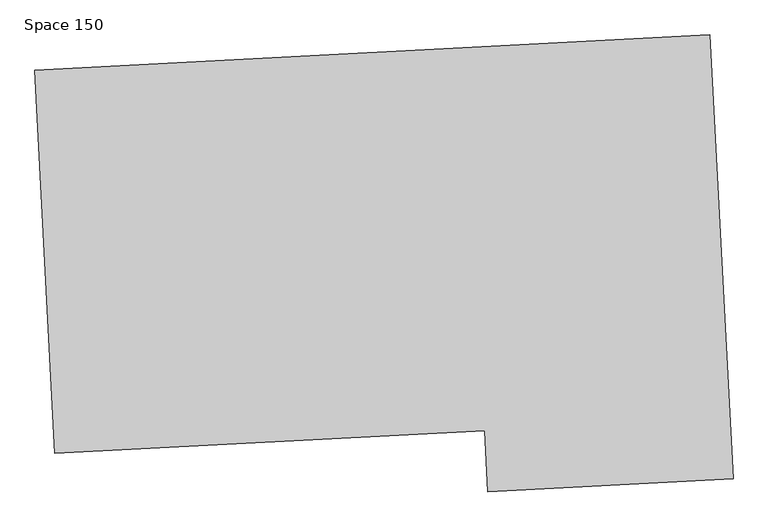
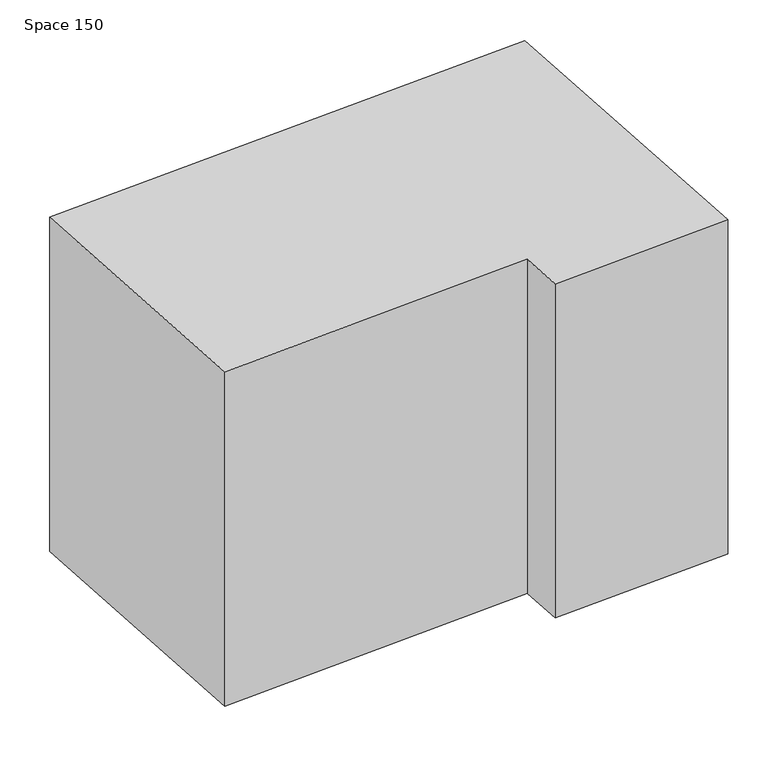
"""IFC4 building model written with IfcOpenShell, lengths in millimetres: proxy geometry, Space 150."""

import ifcopenshell
import ifcopenshell.guid

model = None  # the IFC model being written
_history = None  # IfcOwnerHistory: only IFC2X3 demands one
_inside = {}  # id of a spatial element -> (the spatial element, [elements in it])
_under = {}  # id of a project, library or spatial element -> (it, [spatial elements below it])
_declared = {}  # id of a project -> (the project, [libraries it declares])
_typed = {}  # id of a type object -> (the type object, [elements of that type])
_made_of = {}  # id of a material, layer set ... -> (it, [elements and type objects made of it])


def new_model(schema):
    """Start an empty IFC model of exactly this schema.

    Asked for "IFC4X3", IfcOpenShell would pick the latest addendum, in which some entities
    have other attributes; the version numbers below select the first issue.
    IFC2X3 requires an IfcOwnerHistory on every rooted entity: one is made here for all.
    """
    global model, _history
    if schema == "IFC4X3":
        model = ifcopenshell.file(schema_version=(4, 3, 0, 0))
    else:
        model = ifcopenshell.file(schema=schema)
    _inside.clear()
    _under.clear()
    _declared.clear()
    _typed.clear()
    _made_of.clear()
    _history = None
    if model.schema == "IFC2X3":
        org = make("IfcOrganization", Name="unknown")
        user = make(
            "IfcPersonAndOrganization",
            ThePerson=make("IfcPerson", FamilyName="unknown"),
            TheOrganization=org,
        )
        app = make(
            "IfcApplication",
            ApplicationDeveloper=org,
            Version="unknown",
            ApplicationFullName="unknown",
            ApplicationIdentifier="unknown",
        )
        _history = make(
            "IfcOwnerHistory",
            OwningUser=user,
            OwningApplication=app,
            ChangeAction="ADDED",
            CreationDate=0,
        )
    return model


def make(cls, **values):
    """One entity of the class cls with the attributes given. An attribute that is None is left unset."""
    return model.create_entity(
        cls, **{name: value for name, value in values.items() if value is not None}
    )


def rooted(cls, **values):
    """An entity with a GlobalId (a new one), such as an element, a storey or a relation."""
    return make(cls, GlobalId=ifcopenshell.guid.new(), OwnerHistory=_history, **values)


def si_unit(unit_type, name, prefix=None):
    """IfcSIUnit, for example si_unit("LENGTHUNIT", "METRE", prefix="MILLI")."""
    return make("IfcSIUnit", UnitType=unit_type, Prefix=prefix, Name=name)


def assignment(units):
    """IfcUnitAssignment: the units of a project."""
    return None if units is None else make("IfcUnitAssignment", Units=units)


def point(xyz):
    """IfcCartesianPoint."""
    return None if xyz is None else make("IfcCartesianPoint", Coordinates=xyz)


def direction(xyz):
    """IfcDirection."""
    return None if xyz is None else make("IfcDirection", DirectionRatios=xyz)


def frame(location, z_axis=None, x_axis=None):
    """IfcAxis2Placement3D, a coordinate frame: its origin and axes. An axis left out is left unset."""
    return make(
        "IfcAxis2Placement3D",
        Location=point(location),
        Axis=direction(z_axis),
        RefDirection=direction(x_axis),
    )


def origin():
    """The frame at (0, 0, 0) with its axes left unset."""
    return frame((0.0, 0.0, 0.0))


def place(relative_to, where):
    """IfcLocalPlacement: puts the frame where relative to a parent placement (None: the world)."""
    return make(
        "IfcLocalPlacement", PlacementRelTo=relative_to, RelativePlacement=where
    )


def context(
    kind, dimensions, precision=None, world=None, true_north=None, identifier=None
):
    """IfcGeometricRepresentationContext, for example the 3D "Model" context."""
    return make(
        "IfcGeometricRepresentationContext",
        ContextIdentifier=identifier,
        ContextType=kind,
        CoordinateSpaceDimension=dimensions,
        Precision=precision,
        WorldCoordinateSystem=world,
        TrueNorth=true_north,
    )


def project(units=None, contexts=None):
    """IfcProject with its units and contexts."""
    return rooted(
        "IfcProject",
        Name="project",
        RepresentationContexts=contexts,
        UnitsInContext=assignment(units),
    )


def spatial(cls, under=None, at=None, **own):
    """A site, building, storey or space (cls), placed at a placement, below another one or the project."""
    s = rooted(cls, ObjectPlacement=at, **own)
    if under is not None:
        _under.setdefault(under.id(), (under, []))[1].append(s)
    return s


def polyline(points):
    """IfcPolyline through the points."""
    return make("IfcPolyline", Points=[point(p) for p in points])


def outline(outer, holes=None, kind="AREA"):
    """IfcArbitraryClosedProfileDef: a profile drawn as a closed curve; with holes, ...WithVoids."""
    if holes is None:
        return make("IfcArbitraryClosedProfileDef", ProfileType=kind, OuterCurve=outer)
    return make(
        "IfcArbitraryProfileDefWithVoids",
        ProfileType=kind,
        OuterCurve=outer,
        InnerCurves=holes,
    )


def extrude(swept, where, along, depth):
    """IfcExtrudedAreaSolid: the profile swept, set in the frame where, extruded along a direction by depth."""
    return make(
        "IfcExtrudedAreaSolid",
        SweptArea=swept,
        Position=where,
        ExtrudedDirection=direction(along),
        Depth=depth,
    )


def shape(context_of_items, identifier, shape_type, items):
    """IfcShapeRepresentation: the items that make up one representation, for example the "Body"."""
    return make(
        "IfcShapeRepresentation",
        ContextOfItems=context_of_items,
        RepresentationIdentifier=identifier,
        RepresentationType=shape_type,
        Items=items,
    )


def source(mapping_origin, context_of_items, identifier, shape_type, items):
    """IfcRepresentationMap: a shape defined once, which mapped items show again and again."""
    return make(
        "IfcRepresentationMap",
        MappingOrigin=mapping_origin,
        MappedRepresentation=shape(context_of_items, identifier, shape_type, items),
    )


def transform(
    local_origin,
    x_axis=None,
    y_axis=None,
    z_axis=None,
    scale=None,
    scale2=None,
    scale3=None,
    uniform=True,
):
    """IfcCartesianTransformationOperator3D, or its non-uniform kind. x_axis, y_axis, z_axis: its Axis1, 2, 3."""
    if uniform:
        return make(
            "IfcCartesianTransformationOperator3D",
            Axis1=direction(x_axis),
            Axis2=direction(y_axis),
            LocalOrigin=point(local_origin),
            Scale=scale,
            Axis3=direction(z_axis),
        )
    return make(
        "IfcCartesianTransformationOperator3DnonUniform",
        Axis1=direction(x_axis),
        Axis2=direction(y_axis),
        LocalOrigin=point(local_origin),
        Scale=scale,
        Axis3=direction(z_axis),
        Scale2=scale2,
        Scale3=scale3,
    )


def mapped(mapping_source, mapping_target):
    """IfcMappedItem: shows the shape of a source again, moved by a transform."""
    return make(
        "IfcMappedItem", MappingSource=mapping_source, MappingTarget=mapping_target
    )


def made_of(thing, what):
    """Note that an element or type object is made of a material, layer set ...; save() writes the relation."""
    if what is not None:
        _made_of.setdefault(what.id(), (what, []))[1].append(thing)
    return thing


def element(
    cls,
    number,
    at=None,
    inside=None,
    cuts=None,
    type_object=None,
    material=None,
    context=None,
    identifier="Body",
    shape_type=None,
    held_by="IfcProductDefinitionShape",
    body=None,
    shapes=None,
    **own,
):
    """One element of the class cls, such as IfcWall. Its Tag is "e" and its number.

    at: its placement. inside: the storey or other place that contains it. cuts: it is an
    opening in that element (IfcRelVoidsElement). A single representation is given by context,
    identifier, shape_type and body (its items); several are given by shapes. held_by: the class
    of the entity that holds the representations. save() writes the other relations.
    """
    e = rooted(cls, Tag="e%d" % number, ObjectPlacement=at, **own)
    if body is not None:
        shapes = [shape(context, identifier, shape_type, body)]
    if shapes is not None:
        e.Representation = make(held_by, Representations=shapes)
    if inside is not None:
        _inside.setdefault(inside.id(), (inside, []))[1].append(e)
    if cuts is not None:
        rooted(
            "IfcRelVoidsElement", RelatingBuildingElement=cuts, RelatedOpeningElement=e
        )
    if type_object is not None:
        _typed.setdefault(type_object.id(), (type_object, []))[1].append(e)
    return made_of(e, material)


def aggregate(whole, parts):
    """IfcRelAggregates: a whole, such as a stair, and the parts it consists of."""
    return rooted("IfcRelAggregates", RelatingObject=whole, RelatedObjects=parts)


def save(model, path):
    """Write the relations noted so far, then the file.

    IfcRelAggregates (storeys below a building ...), IfcRelContainedInSpatialStructure (elements
    in a storey), IfcRelDefinesByType, IfcRelAssociatesMaterial and IfcRelDeclares: one each for
    every whole, place, type object, material and project.
    """
    for whole, parts in _under.values():
        aggregate(whole, parts)
    for where, things in _inside.values():
        rooted(
            "IfcRelContainedInSpatialStructure",
            RelatedElements=things,
            RelatingStructure=where,
        )
    for kind, things in _typed.values():
        rooted("IfcRelDefinesByType", RelatedObjects=things, RelatingType=kind)
    for what, things in _made_of.values():
        rooted("IfcRelAssociatesMaterial", RelatedObjects=things, RelatingMaterial=what)
    for by, libraries in _declared.values():
        rooted("IfcRelDeclares", RelatingContext=by, RelatedDefinitions=libraries)
    model.write(path)


def space_150_025012b6(model_context):
    return source(origin(), model_context, "Body", "SweptSolid", [
        extrude(outline(polyline([(10897.8188065, -26633.7981205), (9363.2248005, -26714.2227845), (9343.2848012, -26333.7449318), (6654.5746418, -26474.6542603), (6528.952646, -24077.6437881), (10752.2568114, -23856.3097955), (10897.8188065, -26633.7981205)])), frame((0.0, 0.0, 3810.0), z_axis=(0.0, 0.0, 1.0), x_axis=(1.0, 0.0, 0.0)), (0.0, 0.0, 1.0), 3048.0),
    ])


if __name__ == "__main__":
    model = new_model("IFC4")
    model_context = context("Model", 3, world=origin())
    ifc_project = project(units=[si_unit("LENGTHUNIT", "METRE", prefix="MILLI")], contexts=[model_context])
    site = spatial("IfcSite", under=ifc_project)
    building = spatial("IfcBuilding", under=site)
    placement = place(None, origin())
    space_150_shape = space_150_025012b6(model_context)
    element("IfcBuildingElementProxy", 1, Name="Space 150", ObjectType="Space 150", at=placement, inside=building, context=model_context, shape_type="MappedRepresentation", body=[
        mapped(space_150_shape, transform((0.0, 0.0, 0.0), x_axis=(1.0, 0.0, 0.0), y_axis=(0.0, 1.0, 0.0), z_axis=(0.0, 0.0, 1.0))),
    ])
    save(model, "model.ifc")

# Revit data of these elements
# Project information
#   Project Issue Date = "Issue Date"
#   Project Status = "Project Status"
#   Client Name = "Owner"
#   Project Address = "Enter address here"
#   Project Name = "Project Name"
#   Project Number = "Project Number"
# Element 1 (IfcBuildingElementProxy, "Space 150")
#   Materials on its faces: "Render Material 255-255-255"
# Materials
#   "Render Material 255-255-255": class "Unassigned", colour RGB 255 255 255, transparency 0
